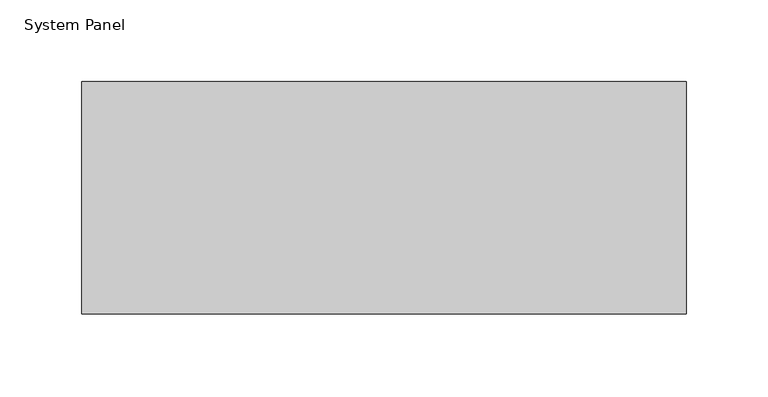
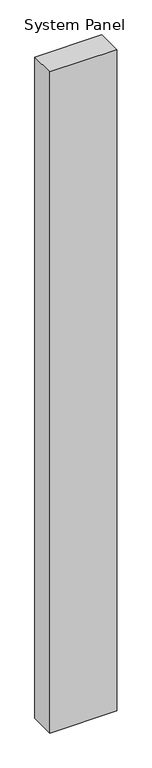
"""IFC4 building model written with IfcOpenShell, lengths in millimetres: plate geometry, System Panel : NLRS_21_CWP_hsb-vulling minerale wol 142 _gen_rsf."""

from ifc_helpers import new_model, si_unit, origin, origin_with_axes, place, context, project, spatial, polyline, outline, extrude, source, transform, mapped, element, save


def system_panel_4b5b3d98(model_context):
    return source(origin(), model_context, "Body", "SweptSolid", [
        extrude(outline(polyline([(184.5, -71.0), (-184.5, -71.0), (-184.5, 71.0), (184.5, 71.0), (184.5, -71.0)])), origin_with_axes(), (0.0, 0.0, 1.0), 3849.0),
    ])


if __name__ == "__main__":
    model = new_model("IFC4")
    model_context = context("Model", 3, world=origin())
    ifc_project = project(units=[si_unit("LENGTHUNIT", "METRE", prefix="MILLI")], contexts=[model_context])
    site = spatial("IfcSite", under=ifc_project)
    building = spatial("IfcBuilding", under=site)
    placement = place(None, origin())
    system_panel_shape = system_panel_4b5b3d98(model_context)
    element("IfcPlate", 1, ObjectType="System Panel : NLRS_21_CWP_hsb-vulling minerale wol 142 _gen_rsf", at=placement, inside=building, context=model_context, shape_type="MappedRepresentation", body=[
        mapped(system_panel_shape, transform((0.0, 0.0, 0.0), x_axis=(1.0, 0.0, 0.0), y_axis=(0.0, 1.0, 0.0), z_axis=(0.0, 0.0, 1.0))),
    ])
    save(model, "model.ifc")

# Revit data of these elements
# Type "System Panel : NLRS_21_CWP_hsb-vulling minerale wol 142 _gen_rsf"
#   Export Type to IFC As = "IfcWall"
#   Type IfcGUID = "07M7mRoiH1CR8m_RSKIwpC"
#   Assembly Code = "21.23"
# Element 1 (IfcPlate, "System Panel : NLRS_21_CWP_hsb-vulling minerale wol 142 _gen_rsf")
#   Materials on its faces: "NLRS_m1_isolatie minerale wol_gen_rsf"
# Materials
#   "NLRS_m1_isolatie minerale wol_gen_rsf": class "M - Anorganische materialen", colour RGB 200 200 140, transparency 0, Keynote = "m1", Manufacturer = "Revit Standards Foundation", URL = "www.revitstandards.org", Description = "isolatie minerale wol", Cost = 0
